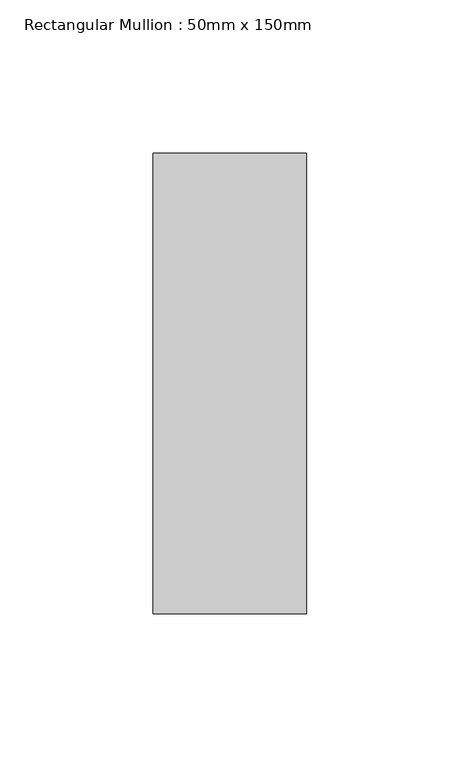
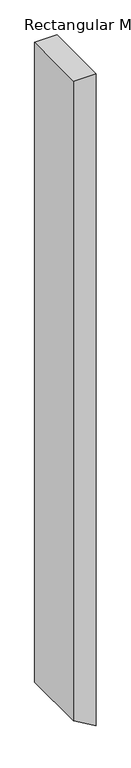
"""IFC4 building model written with IfcOpenShell, lengths in millimetres: member geometry, Rectangular Mullion : 50mm x 150mm."""

from ifc_helpers import new_model, si_unit, frame, origin, place, context, project, spatial, polyline, outline, extrude, source, transform, mapped, element, save


def rectangular_mullion_50mm_x_150mm_ed641c16(model_context):
    return source(origin(), model_context, "Body", "SweptSolid", [
        extrude(outline(polyline([(0.0, 0.0), (0.0, -50.0), (-1505.2346306, -50.0), (-1534.1021441, 0.0), (0.0, 0.0)])), frame((0.0, -75.0, 0.0), z_axis=(0.0, 1.0, 0.0), x_axis=(0.0, 0.0, 1.0)), (0.0, 0.0, 1.0), 150.0),
    ])


if __name__ == "__main__":
    model = new_model("IFC4")
    model_context = context("Model", 3, world=origin())
    ifc_project = project(units=[si_unit("LENGTHUNIT", "METRE", prefix="MILLI")], contexts=[model_context])
    site = spatial("IfcSite", under=ifc_project)
    building = spatial("IfcBuilding", under=site)
    placement = place(None, origin())
    rectangular_mullion_50mm_x_150mm_shape = rectangular_mullion_50mm_x_150mm_ed641c16(model_context)
    element("IfcMember", 1, ObjectType="Rectangular Mullion : 50mm x 150mm", at=placement, inside=building, context=model_context, shape_type="MappedRepresentation", body=[
        mapped(rectangular_mullion_50mm_x_150mm_shape, transform((0.0, 0.0, 0.0), x_axis=(1.0, 0.0, 0.0), y_axis=(0.0, 1.0, 0.0), z_axis=(0.0, 0.0, 1.0))),
    ])
    save(model, "model.ifc")

# Revit data of these elements
# Type "Rectangular Mullion : 50mm x 150mm"
#   built-in parameter 1007304 = 0.492126 (stored number, unit not read)
#   built-in parameter 1007301 = 0.082021 (stored number, unit not read)
#   built-in parameter 1007300 = 0.082021 (stored number, unit not read)
# Element 1 (IfcMember, "Rectangular Mullion : 50mm x 150mm")
#   Materials on its faces: "Aluminum"
# Materials
#   "Aluminum": class "Metal", colour RGB 247 247 247, transparency 0, Description = "Aluminum 6061", Cost = 0
